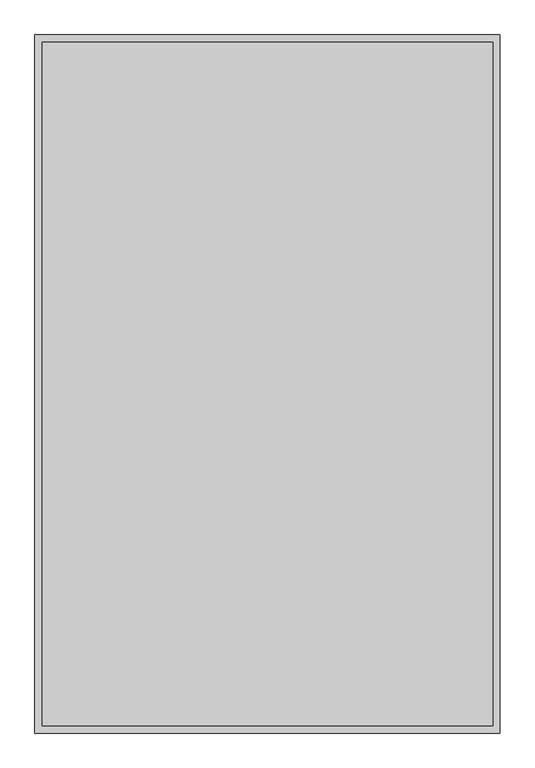
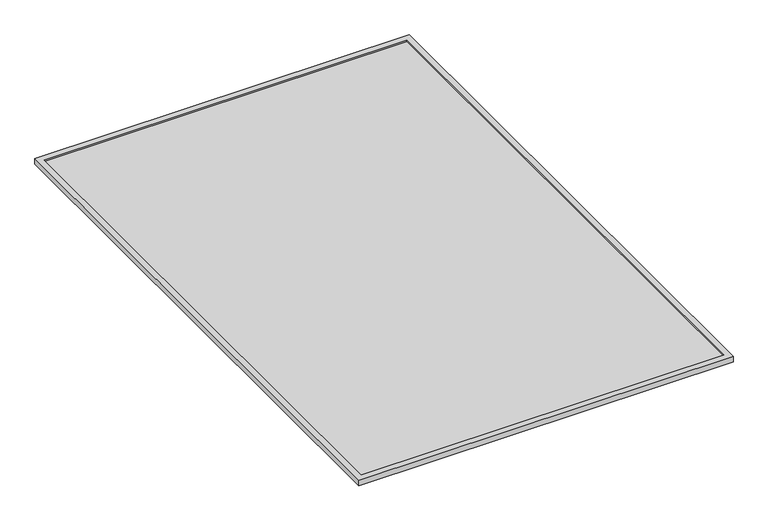
"""IFC4 building model written with IfcOpenShell, lengths in millimetres: proxy geometry, Bradley-Washroom_Accessories-Mirrors-780_Custom : Bradley-Washroom_Accessories-Mirrors-780_Custom."""

from ifc_helpers import new_model, si_unit, frame, origin, place, context, project, spatial, polyline, outline, extrude, faceted_brep, source, transform, mapped, element, save


def specialty_equipment_8c61682c(model_context):
    return source(origin(), model_context, "Body", "SolidModel", [
        extrude(outline(polyline([(590.55, 895.35), (590.55, -895.35), (-590.55, -895.35), (-590.55, 895.35), (590.55, 895.35)])), frame((0.0, 0.0, 9.525), z_axis=(0.0, 0.0, 1.0), x_axis=(1.0, 0.0, 0.0)), (0.0, 0.0, 1.0), 4.7625),
        faceted_brep([(609.6, 914.4, 19.05), (-609.6, 914.4, 19.05), (-609.6, -914.4, 19.05), (609.6, -914.4, 19.05), (-590.55, 895.35, 19.05), (590.55, 895.35, 19.05), (590.55, -895.35, 19.05), (-590.55, -895.35, 19.05), (609.6, 914.4, 0.0), (609.6, -914.4, 0.0), (-609.6, -914.4, 0.0), (-609.6, 914.4, 0.0), (590.55, 895.35, 9.525), (-590.55, 895.35, 9.525), (-590.55, -895.35, 9.525), (590.55, -895.35, 9.525)], [[[0, 1, 2, 3], [4, 5, 6, 7]], [[8, 9, 10, 11]], [[1, 0, 8, 11]], [[2, 1, 11, 10]], [[3, 2, 10, 9]], [[0, 3, 9, 8]], [[12, 13, 14, 15]], [[13, 12, 5, 4]], [[14, 13, 4, 7]], [[15, 14, 7, 6]], [[12, 15, 6, 5]]]),
    ])


if __name__ == "__main__":
    model = new_model("IFC4")
    model_context = context("Model", 3, world=origin())
    ifc_project = project(units=[si_unit("LENGTHUNIT", "METRE", prefix="MILLI")], contexts=[model_context])
    site = spatial("IfcSite", under=ifc_project)
    building = spatial("IfcBuilding", under=site)
    placement = place(None, origin())
    specialty_equipment_shape = specialty_equipment_8c61682c(model_context)
    element("IfcBuildingElementProxy", 1, Name="Bradley-Washroom_Accessories-Mirrors-780_Custom : Bradley-Washroom_Accessories-Mirrors-780_Custom", ObjectType="Bradley-Washroom_Accessories-Mirrors-780_Custom : Bradley-Washroom_Accessories-Mirrors-780_Custom", at=placement, inside=building, context=model_context, shape_type="MappedRepresentation", body=[
        mapped(specialty_equipment_shape, transform((0.0, 0.0, 0.0), x_axis=(1.0, 0.0, 0.0), y_axis=(0.0, 1.0, 0.0), z_axis=(0.0, 0.0, 1.0))),
    ])
    save(model, "model.ifc")

# Revit data of these elements
# Type "Bradley-Washroom_Accessories-Mirrors-780_Custom : Bradley-Washroom_Accessories-Mirrors-780_Custom"
#   Keynote = "M08831300.01"
#   Warranty Information = "Complete unit, excepting mirrors warranted for one year.\r\n Stainless steel mirror frames for fifteen years.\r\n Plate glass mirrors for fifteen years.\r\n This warranty does not cover installation or any other labor charges and does not apply to any units,\r\n which have been damaged by accident, abuse, improper installation, improper maintenance, or altered in any way."
#   Version = "1.0"
#   URL = "http://www.bradleycorp.com/"
#   Type Comments = "ERROR - If you are able to see this message you haven't loaded this  family correctly."
#   OmniClass Title = "Mirrors"
#   OmniClass Code = "23.40.95.17.17"
#   Modeling Code = ""
#   Model = "ERROR - If you are able to see this message you haven't loaded this  family correctly."
#   MasterFormat Title = "Commercial Toilet Accessories"
#   MasterFormat Number = "10 28 13. 13"
#   Manufacturer = "Bradley Corporation"
#   Industry Standards = "ASTM C 1036"
#   Fire Rating = "n/a"
#   Dimensional Limits [instance default] = "Either Width or Hight must be over 25\""
#   Description = "ERROR - If you are able to see this message you haven't loaded this  family correctly."
#   Copyright = "This Model Data is Property of Bradley Corporation"
#   Buy American Act = "Yes"
#   Assembly Code = "C1030900"
#   ADA Compliant = "Yes"
#   Width [instance default] = 1' - 6"
#   Total Width [instance default] = 1' - 6"
#   Total Height [instance default] = 3' - 0"
#   Height [instance default] = 3' - 0"
#   Depth [instance default] = 0' - 0 3/4"
#   Default Elevation = 3' - 4"
#   Reflective Material = Glass - Bradley Corp - BradEX - Polished Float Mirror
#   Frame Material = Bradley Corp Stainless Steel - Satin
# Element 1 (IfcBuildingElementProxy, "Bradley-Washroom_Accessories-Mirrors-780_Custom : Bradley-Washroom_Accessories-Mirrors-780_Custom")
#   Width = 4' - 0"
#   Total Width = 4' - 0"
#   Total Height = 6' - 0"
#   Height = 6' - 0"
#   Materials on its faces: "Bradley Corp Stainless Steel - Satin", "Glass - Bradley Corp - BradEX - Polished Float Mirror"
# Materials
#   "Glass - Bradley Corp - BradEX - Polished Float Mirror": class "Glass", colour RGB 221 230 232, transparency 0, Manufacturer = "Bradley Corporation", URL = "www.bradleycorp.com", Description = "Stainless Steel - Satin Finish", Cost = 0
#   "Bradley Corp Stainless Steel - Satin": class "Metal", colour RGB 189 187 185, transparency 0, Manufacturer = "Bradley Corporation", URL = "www.bradleycorp.com", Description = "Stainless Steel - Satin Finish", Cost = 0
